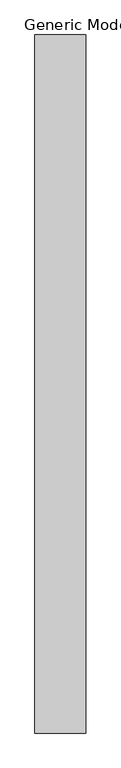
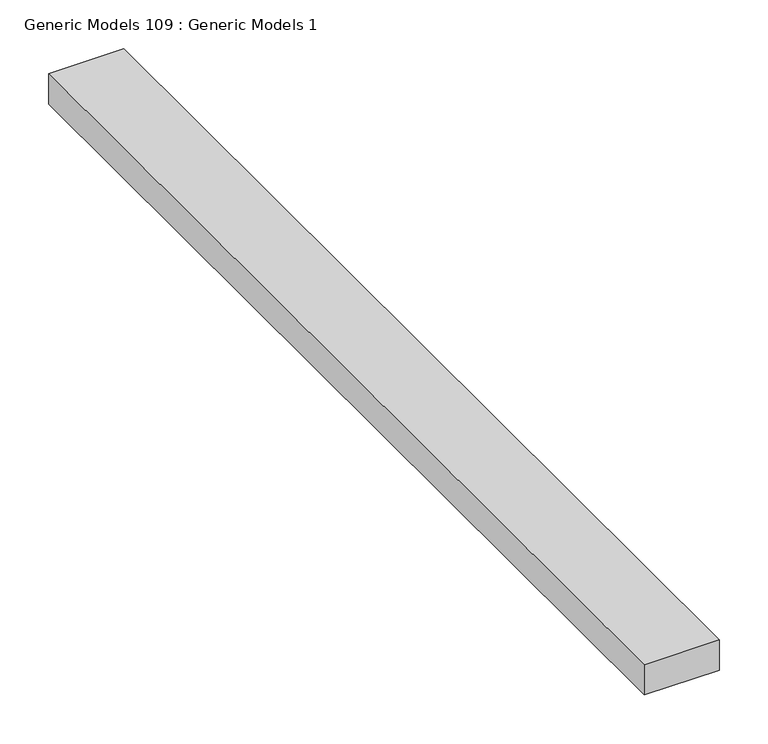
"""IFC4 building model written with IfcOpenShell, lengths in millimetres: proxy geometry, Generic Models 109 : Generic Models 1."""

import ifcopenshell
import ifcopenshell.guid

model = None  # the IFC model being written
_history = None  # IfcOwnerHistory: only IFC2X3 demands one
_inside = {}  # id of a spatial element -> (the spatial element, [elements in it])
_under = {}  # id of a project, library or spatial element -> (it, [spatial elements below it])
_declared = {}  # id of a project -> (the project, [libraries it declares])
_typed = {}  # id of a type object -> (the type object, [elements of that type])
_made_of = {}  # id of a material, layer set ... -> (it, [elements and type objects made of it])


def new_model(schema):
    """Start an empty IFC model of exactly this schema.

    Asked for "IFC4X3", IfcOpenShell would pick the latest addendum, in which some entities
    have other attributes; the version numbers below select the first issue.
    IFC2X3 requires an IfcOwnerHistory on every rooted entity: one is made here for all.
    """
    global model, _history
    if schema == "IFC4X3":
        model = ifcopenshell.file(schema_version=(4, 3, 0, 0))
    else:
        model = ifcopenshell.file(schema=schema)
    _inside.clear()
    _under.clear()
    _declared.clear()
    _typed.clear()
    _made_of.clear()
    _history = None
    if model.schema == "IFC2X3":
        org = make("IfcOrganization", Name="unknown")
        user = make(
            "IfcPersonAndOrganization",
            ThePerson=make("IfcPerson", FamilyName="unknown"),
            TheOrganization=org,
        )
        app = make(
            "IfcApplication",
            ApplicationDeveloper=org,
            Version="unknown",
            ApplicationFullName="unknown",
            ApplicationIdentifier="unknown",
        )
        _history = make(
            "IfcOwnerHistory",
            OwningUser=user,
            OwningApplication=app,
            ChangeAction="ADDED",
            CreationDate=0,
        )
    return model


def make(cls, **values):
    """One entity of the class cls with the attributes given. An attribute that is None is left unset."""
    return model.create_entity(
        cls, **{name: value for name, value in values.items() if value is not None}
    )


def rooted(cls, **values):
    """An entity with a GlobalId (a new one), such as an element, a storey or a relation."""
    return make(cls, GlobalId=ifcopenshell.guid.new(), OwnerHistory=_history, **values)


def si_unit(unit_type, name, prefix=None):
    """IfcSIUnit, for example si_unit("LENGTHUNIT", "METRE", prefix="MILLI")."""
    return make("IfcSIUnit", UnitType=unit_type, Prefix=prefix, Name=name)


def assignment(units):
    """IfcUnitAssignment: the units of a project."""
    return None if units is None else make("IfcUnitAssignment", Units=units)


def point(xyz):
    """IfcCartesianPoint."""
    return None if xyz is None else make("IfcCartesianPoint", Coordinates=xyz)


def direction(xyz):
    """IfcDirection."""
    return None if xyz is None else make("IfcDirection", DirectionRatios=xyz)


def frame(location, z_axis=None, x_axis=None):
    """IfcAxis2Placement3D, a coordinate frame: its origin and axes. An axis left out is left unset."""
    return make(
        "IfcAxis2Placement3D",
        Location=point(location),
        Axis=direction(z_axis),
        RefDirection=direction(x_axis),
    )


def origin():
    """The frame at (0, 0, 0) with its axes left unset."""
    return frame((0.0, 0.0, 0.0))


def place(relative_to, where):
    """IfcLocalPlacement: puts the frame where relative to a parent placement (None: the world)."""
    return make(
        "IfcLocalPlacement", PlacementRelTo=relative_to, RelativePlacement=where
    )


def context(
    kind, dimensions, precision=None, world=None, true_north=None, identifier=None
):
    """IfcGeometricRepresentationContext, for example the 3D "Model" context."""
    return make(
        "IfcGeometricRepresentationContext",
        ContextIdentifier=identifier,
        ContextType=kind,
        CoordinateSpaceDimension=dimensions,
        Precision=precision,
        WorldCoordinateSystem=world,
        TrueNorth=true_north,
    )


def project(units=None, contexts=None):
    """IfcProject with its units and contexts."""
    return rooted(
        "IfcProject",
        Name="project",
        RepresentationContexts=contexts,
        UnitsInContext=assignment(units),
    )


def spatial(cls, under=None, at=None, **own):
    """A site, building, storey or space (cls), placed at a placement, below another one or the project."""
    s = rooted(cls, ObjectPlacement=at, **own)
    if under is not None:
        _under.setdefault(under.id(), (under, []))[1].append(s)
    return s


def polyline(points):
    """IfcPolyline through the points."""
    return make("IfcPolyline", Points=[point(p) for p in points])


def outline(outer, holes=None, kind="AREA"):
    """IfcArbitraryClosedProfileDef: a profile drawn as a closed curve; with holes, ...WithVoids."""
    if holes is None:
        return make("IfcArbitraryClosedProfileDef", ProfileType=kind, OuterCurve=outer)
    return make(
        "IfcArbitraryProfileDefWithVoids",
        ProfileType=kind,
        OuterCurve=outer,
        InnerCurves=holes,
    )


def extrude(swept, where, along, depth):
    """IfcExtrudedAreaSolid: the profile swept, set in the frame where, extruded along a direction by depth."""
    return make(
        "IfcExtrudedAreaSolid",
        SweptArea=swept,
        Position=where,
        ExtrudedDirection=direction(along),
        Depth=depth,
    )


def shape(context_of_items, identifier, shape_type, items):
    """IfcShapeRepresentation: the items that make up one representation, for example the "Body"."""
    return make(
        "IfcShapeRepresentation",
        ContextOfItems=context_of_items,
        RepresentationIdentifier=identifier,
        RepresentationType=shape_type,
        Items=items,
    )


def source(mapping_origin, context_of_items, identifier, shape_type, items):
    """IfcRepresentationMap: a shape defined once, which mapped items show again and again."""
    return make(
        "IfcRepresentationMap",
        MappingOrigin=mapping_origin,
        MappedRepresentation=shape(context_of_items, identifier, shape_type, items),
    )


def transform(
    local_origin,
    x_axis=None,
    y_axis=None,
    z_axis=None,
    scale=None,
    scale2=None,
    scale3=None,
    uniform=True,
):
    """IfcCartesianTransformationOperator3D, or its non-uniform kind. x_axis, y_axis, z_axis: its Axis1, 2, 3."""
    if uniform:
        return make(
            "IfcCartesianTransformationOperator3D",
            Axis1=direction(x_axis),
            Axis2=direction(y_axis),
            LocalOrigin=point(local_origin),
            Scale=scale,
            Axis3=direction(z_axis),
        )
    return make(
        "IfcCartesianTransformationOperator3DnonUniform",
        Axis1=direction(x_axis),
        Axis2=direction(y_axis),
        LocalOrigin=point(local_origin),
        Scale=scale,
        Axis3=direction(z_axis),
        Scale2=scale2,
        Scale3=scale3,
    )


def mapped(mapping_source, mapping_target):
    """IfcMappedItem: shows the shape of a source again, moved by a transform."""
    return make(
        "IfcMappedItem", MappingSource=mapping_source, MappingTarget=mapping_target
    )


def made_of(thing, what):
    """Note that an element or type object is made of a material, layer set ...; save() writes the relation."""
    if what is not None:
        _made_of.setdefault(what.id(), (what, []))[1].append(thing)
    return thing


def element(
    cls,
    number,
    at=None,
    inside=None,
    cuts=None,
    type_object=None,
    material=None,
    context=None,
    identifier="Body",
    shape_type=None,
    held_by="IfcProductDefinitionShape",
    body=None,
    shapes=None,
    **own,
):
    """One element of the class cls, such as IfcWall. Its Tag is "e" and its number.

    at: its placement. inside: the storey or other place that contains it. cuts: it is an
    opening in that element (IfcRelVoidsElement). A single representation is given by context,
    identifier, shape_type and body (its items); several are given by shapes. held_by: the class
    of the entity that holds the representations. save() writes the other relations.
    """
    e = rooted(cls, Tag="e%d" % number, ObjectPlacement=at, **own)
    if body is not None:
        shapes = [shape(context, identifier, shape_type, body)]
    if shapes is not None:
        e.Representation = make(held_by, Representations=shapes)
    if inside is not None:
        _inside.setdefault(inside.id(), (inside, []))[1].append(e)
    if cuts is not None:
        rooted(
            "IfcRelVoidsElement", RelatingBuildingElement=cuts, RelatedOpeningElement=e
        )
    if type_object is not None:
        _typed.setdefault(type_object.id(), (type_object, []))[1].append(e)
    return made_of(e, material)


def aggregate(whole, parts):
    """IfcRelAggregates: a whole, such as a stair, and the parts it consists of."""
    return rooted("IfcRelAggregates", RelatingObject=whole, RelatedObjects=parts)


def save(model, path):
    """Write the relations noted so far, then the file.

    IfcRelAggregates (storeys below a building ...), IfcRelContainedInSpatialStructure (elements
    in a storey), IfcRelDefinesByType, IfcRelAssociatesMaterial and IfcRelDeclares: one each for
    every whole, place, type object, material and project.
    """
    for whole, parts in _under.values():
        aggregate(whole, parts)
    for where, things in _inside.values():
        rooted(
            "IfcRelContainedInSpatialStructure",
            RelatedElements=things,
            RelatingStructure=where,
        )
    for kind, things in _typed.values():
        rooted("IfcRelDefinesByType", RelatedObjects=things, RelatingType=kind)
    for what, things in _made_of.values():
        rooted("IfcRelAssociatesMaterial", RelatedObjects=things, RelatingMaterial=what)
    for by, libraries in _declared.values():
        rooted("IfcRelDeclares", RelatingContext=by, RelatedDefinitions=libraries)
    model.write(path)


def generic_models_109_generic_models_1_8619d77b(model_context):
    return source(origin(), model_context, "Body", "SweptSolid", [
        extrude(outline(polyline([(51003.2, 0.0), (50914.3, 0.0), (50914.3, 1219.2), (51003.2, 1219.2), (51003.2, 0.0)])), frame((0.0, 0.0, 5184.378125), z_axis=(0.0, 0.0, 1.0), x_axis=(1.0, 0.0, 0.0)), (0.0, 0.0, 1.0), 38.1),
    ])


if __name__ == "__main__":
    model = new_model("IFC4")
    model_context = context("Model", 3, world=origin())
    ifc_project = project(units=[si_unit("LENGTHUNIT", "METRE", prefix="MILLI")], contexts=[model_context])
    site = spatial("IfcSite", under=ifc_project)
    building = spatial("IfcBuilding", under=site)
    placement = place(None, origin())
    generic_models_109_generic_models_1_shape = generic_models_109_generic_models_1_8619d77b(model_context)
    element("IfcBuildingElementProxy", 1, Name="Generic Models 109 : Generic Models 1", ObjectType="Generic Models 109 : Generic Models 1", at=placement, inside=building, context=model_context, shape_type="MappedRepresentation", body=[
        mapped(generic_models_109_generic_models_1_shape, transform((0.0, 0.0, 0.0), x_axis=(1.0, 0.0, 0.0), y_axis=(0.0, 1.0, 0.0), z_axis=(0.0, 0.0, 1.0))),
    ])
    save(model, "model.ifc")

# Revit data of these elements
# Element 1 (IfcBuildingElementProxy, "Generic Models 109 : Generic Models 1")
#   Materials on its faces: "DOUBLE 2X WOOD TOP PLATE"
# Materials
#   "DOUBLE 2X WOOD TOP PLATE": class "Wood", colour RGB 234 198 147, transparency 0, Description = "Pinus Echinata", Cost = 0
